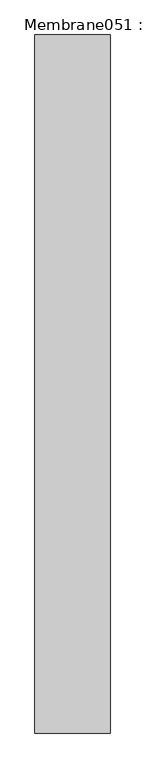
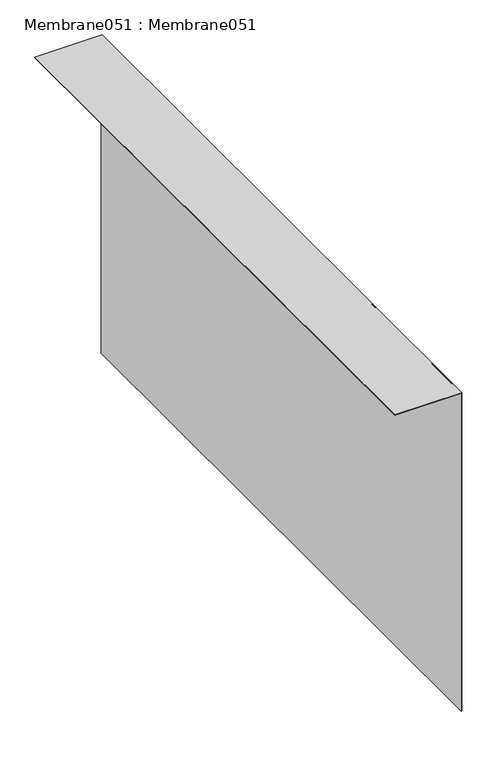
"""IFC4 building model written with IfcOpenShell, lengths in millimetres: proxy geometry, Membrane051 : Membrane051."""

from ifc_helpers import new_model, si_unit, frame, origin, place, context, project, spatial, polyline, outline, extrude, source, transform, mapped, element, save


def membrane051_membrane051_90222649(model_context):
    return source(origin(), model_context, "Body", "SweptSolid", [
        extrude(outline(polyline([(33391.6445312, -10088.4443359), (32314.8961275, -10088.4443359), (32314.8961275, -10086.4443359), (33393.6445312, -10086.4443359), (33393.6445312, -10301.6737014), (33391.6445312, -10301.6737014), (33391.6445312, -10088.4443359)])), frame((0.0, 7182.1531721, 0.0), z_axis=(0.0, 1.0, 0.0), x_axis=(0.0, 0.0, 1.0)), (0.0, 0.0, 1.0), 2000.0),
    ])


if __name__ == "__main__":
    model = new_model("IFC4")
    model_context = context("Model", 3, world=origin())
    ifc_project = project(units=[si_unit("LENGTHUNIT", "METRE", prefix="MILLI")], contexts=[model_context])
    site = spatial("IfcSite", under=ifc_project)
    building = spatial("IfcBuilding", under=site)
    placement = place(None, origin())
    membrane051_membrane051_shape = membrane051_membrane051_90222649(model_context)
    element("IfcBuildingElementProxy", 1, Name="Membrane051 : Membrane051", ObjectType="Membrane051 : Membrane051", at=placement, inside=building, context=model_context, shape_type="MappedRepresentation", body=[
        mapped(membrane051_membrane051_shape, transform((0.0, 0.0, 0.0), x_axis=(1.0, 0.0, 0.0), y_axis=(0.0, 1.0, 0.0), z_axis=(0.0, 0.0, 1.0))),
    ])
    save(model, "model.ifc")

# Revit data of these elements
# Type "Membrane051 : Membrane051"
#   NameOverride = "Membrane051"
# Element 1 (IfcBuildingElementProxy, "Membrane051 : Membrane051")
#   Materials on its faces: "ECO ROOT BARRIER"
# Materials
#   "ECO ROOT BARRIER": class "Unassigned", colour RGB 135 255 2, transparency 0
